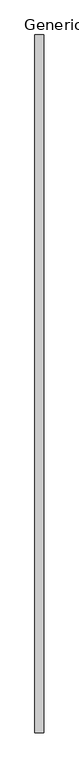
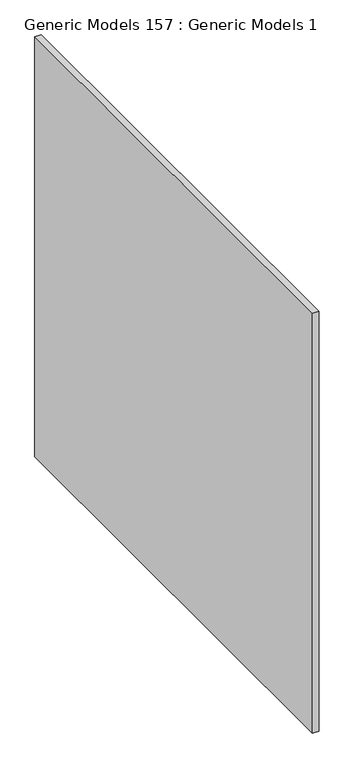
"""IFC4 building model written with IfcOpenShell, lengths in millimetres: proxy geometry, Generic Models 157 : Generic Models 1."""

from ifc_helpers import new_model, si_unit, frame, origin, place, context, project, spatial, polyline, outline, extrude, source, transform, mapped, element, save


def generic_models_157_generic_models_1_b3b9a6c0(model_context):
    return source(origin(), model_context, "Body", "SweptSolid", [
        extrude(outline(polyline([(47363.0625, 1219.2), (47363.0625, 0.0), (47347.1875, 0.0), (47347.1875, 1219.2), (47363.0625, 1219.2)])), frame((0.0, 0.0, 4267.2), z_axis=(0.0, 0.0, 1.0), x_axis=(1.0, 0.0, 0.0)), (0.0, 0.0, 1.0), 1123.95),
    ])


if __name__ == "__main__":
    model = new_model("IFC4")
    model_context = context("Model", 3, world=origin())
    ifc_project = project(units=[si_unit("LENGTHUNIT", "METRE", prefix="MILLI")], contexts=[model_context])
    site = spatial("IfcSite", under=ifc_project)
    building = spatial("IfcBuilding", under=site)
    placement = place(None, origin())
    generic_models_157_generic_models_1_shape = generic_models_157_generic_models_1_b3b9a6c0(model_context)
    element("IfcBuildingElementProxy", 1, Name="Generic Models 157 : Generic Models 1", ObjectType="Generic Models 157 : Generic Models 1", at=placement, inside=building, context=model_context, shape_type="MappedRepresentation", body=[
        mapped(generic_models_157_generic_models_1_shape, transform((0.0, 0.0, 0.0), x_axis=(1.0, 0.0, 0.0), y_axis=(0.0, 1.0, 0.0), z_axis=(0.0, 0.0, 1.0))),
    ])
    save(model, "model.ifc")

# Revit data of these elements
# Element 1 (IfcBuildingElementProxy, "Generic Models 157 : Generic Models 1")
#   Materials on its faces: "GYP. BD (SEE 'WALL TAG' & 'LAYER MATERIAL SCHEDULE' FOR DETAILS)"
# Materials
#   "GYP. BD (SEE 'WALL TAG' & 'LAYER MATERIAL SCHEDULE' FOR DETAILS)": class "Generic", colour RGB 237 236 233, transparency 0, Description = "Gypsum Wall Board", Cost = 0
